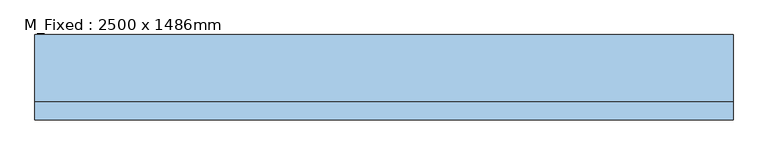
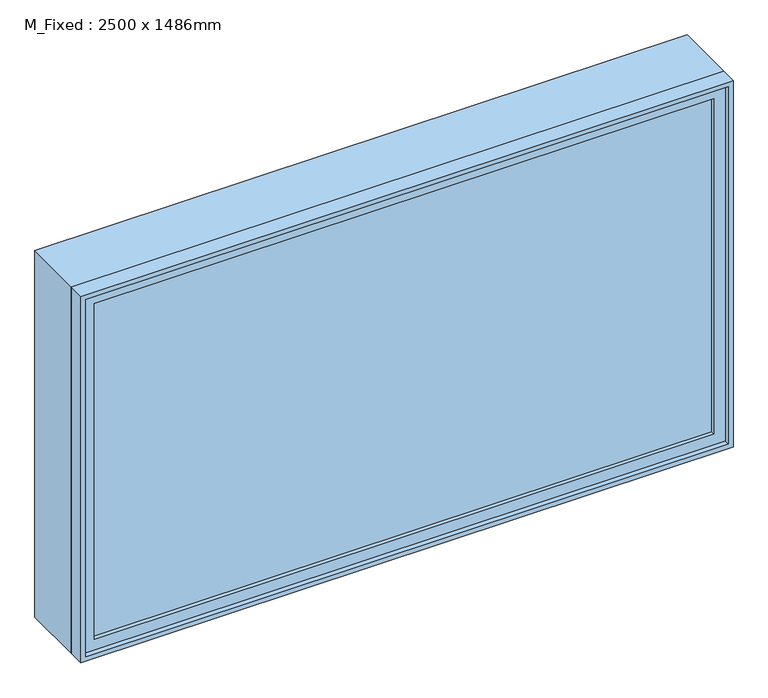
"""IFC4 building model written with IfcOpenShell, lengths in millimetres: window geometry, M_Fixed : 2500 x 1486mm."""

from ifc_helpers import new_model, si_unit, frame, origin, place, context, project, spatial, polyline, outline, extrude, source, transform, mapped, element, save


def m_fixed_2500_x_1486mm_49bc14c1(model_context):
    return source(origin(), model_context, "Body", "SweptSolid", [
        extrude(outline(polyline([(-1187.0, -130.4), (-1187.0, -118.4), (1187.0, -118.4), (1187.0, -130.4), (-1187.0, -130.4)])), frame((0.0, 0.0, 978.0), z_axis=(0.0, 0.0, 1.0), x_axis=(1.0, 0.0, 0.0)), (0.0, 0.0, 1.0), 1360.5),
        extrude(outline(polyline([(2382.5, -1231.0), (934.0, -1231.0), (934.0, 1231.0), (2382.5, 1231.0), (2382.5, -1231.0)]), holes=[polyline([(2338.5, -1187.0), (2338.5, 1187.0), (978.0, 1187.0), (978.0, -1187.0), (2338.5, -1187.0)])]), frame((0.0, -146.4, 0.0), z_axis=(0.0, 1.0, 0.0), x_axis=(0.0, 0.0, 1.0)), (0.0, 0.0, 1.0), 44.0),
        extrude(outline(polyline([(2401.5, -1250.0), (915.0, -1250.0), (915.0, 1250.0), (2401.5, 1250.0), (2401.5, -1250.0)]), holes=[polyline([(2382.5, -1231.0), (2382.5, 1231.0), (934.0, 1231.0), (934.0, -1231.0), (2382.5, -1231.0)])]), frame((0.0, -165.4, 0.0), z_axis=(0.0, 1.0, 0.0), x_axis=(0.0, 0.0, 1.0)), (0.0, 0.0, 1.0), 63.0),
        extrude(outline(polyline([(2401.5, -1250.0), (915.0, -1250.0), (915.0, 1250.0), (2401.5, 1250.0), (2401.5, -1250.0)]), holes=[polyline([(2369.5, -1218.0), (2369.5, 1218.0), (947.0, 1218.0), (947.0, -1218.0), (2369.5, -1218.0)])]), frame((0.0, -102.4, 0.0), z_axis=(0.0, 1.0, 0.0), x_axis=(0.0, 0.0, 1.0)), (0.0, 0.0, 1.0), 241.8),
    ])


if __name__ == "__main__":
    model = new_model("IFC4")
    model_context = context("Model", 3, world=origin())
    ifc_project = project(units=[si_unit("LENGTHUNIT", "METRE", prefix="MILLI")], contexts=[model_context])
    site = spatial("IfcSite", under=ifc_project)
    building = spatial("IfcBuilding", under=site)
    placement = place(None, origin())
    m_fixed_2500_x_1486mm_shape = m_fixed_2500_x_1486mm_49bc14c1(model_context)
    element("IfcWindow", 1, ObjectType="M_Fixed : 2500 x 1486mm", at=placement, inside=building, context=model_context, shape_type="MappedRepresentation", body=[
        mapped(m_fixed_2500_x_1486mm_shape, transform((0.0, 0.0, 0.0), x_axis=(1.0, 0.0, 0.0), y_axis=(0.0, 1.0, 0.0), z_axis=(0.0, 0.0, 1.0))),
    ])
    save(model, "model.ifc")

# Revit data of these elements
# Type "M_Fixed : 2500 x 1486mm"
#   Type Mark = "19"
#   Height = 1486.5 mm
#   Default Sill Height = 915 mm
#   Width = 2500 mm
#   Window Inset = 19 mm
#   Frame Exterior Material = Sash
#   Frame Interior Material = Sash
#   Glass Pane Material = Glass
#   Sash = Sash
#   Wall Closure = (empty or 0)
# Element 1 (IfcWindow, "M_Fixed : 2500 x 1486mm")
#   Materials on its faces: "Sash", "Glass"
# Materials
#   "Sash": class "Wood", colour RGB 136 99 55, transparency 0
#   "Glass": class "Glass", colour RGB 0 128 192, transparency 0.9, Description = "Soda Lime Glass", Cost = 0
